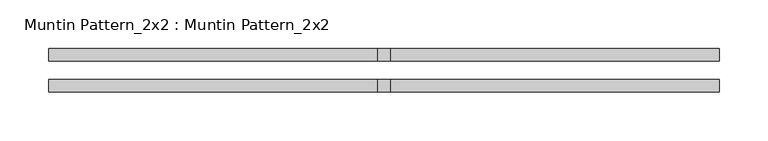
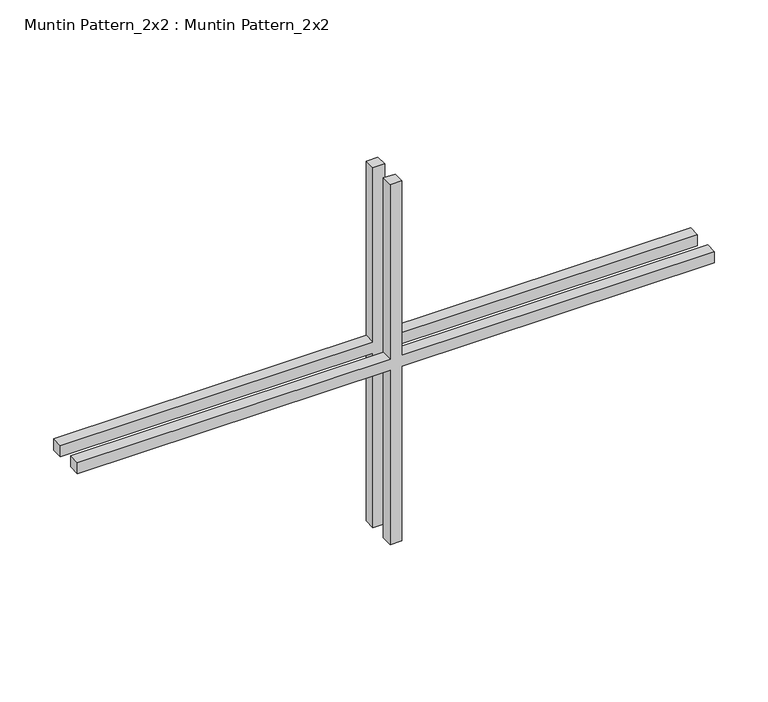
"""IFC4 building model written with IfcOpenShell, lengths in millimetres: proxy geometry, Muntin Pattern_2x2 : Muntin Pattern_2x2."""

import ifcopenshell
import ifcopenshell.guid

model = None  # the IFC model being written
_history = None  # IfcOwnerHistory: only IFC2X3 demands one
_inside = {}  # id of a spatial element -> (the spatial element, [elements in it])
_under = {}  # id of a project, library or spatial element -> (it, [spatial elements below it])
_declared = {}  # id of a project -> (the project, [libraries it declares])
_typed = {}  # id of a type object -> (the type object, [elements of that type])
_made_of = {}  # id of a material, layer set ... -> (it, [elements and type objects made of it])


def new_model(schema):
    """Start an empty IFC model of exactly this schema.

    Asked for "IFC4X3", IfcOpenShell would pick the latest addendum, in which some entities
    have other attributes; the version numbers below select the first issue.
    IFC2X3 requires an IfcOwnerHistory on every rooted entity: one is made here for all.
    """
    global model, _history
    if schema == "IFC4X3":
        model = ifcopenshell.file(schema_version=(4, 3, 0, 0))
    else:
        model = ifcopenshell.file(schema=schema)
    _inside.clear()
    _under.clear()
    _declared.clear()
    _typed.clear()
    _made_of.clear()
    _history = None
    if model.schema == "IFC2X3":
        org = make("IfcOrganization", Name="unknown")
        user = make(
            "IfcPersonAndOrganization",
            ThePerson=make("IfcPerson", FamilyName="unknown"),
            TheOrganization=org,
        )
        app = make(
            "IfcApplication",
            ApplicationDeveloper=org,
            Version="unknown",
            ApplicationFullName="unknown",
            ApplicationIdentifier="unknown",
        )
        _history = make(
            "IfcOwnerHistory",
            OwningUser=user,
            OwningApplication=app,
            ChangeAction="ADDED",
            CreationDate=0,
        )
    return model


def make(cls, **values):
    """One entity of the class cls with the attributes given. An attribute that is None is left unset."""
    return model.create_entity(
        cls, **{name: value for name, value in values.items() if value is not None}
    )


def rooted(cls, **values):
    """An entity with a GlobalId (a new one), such as an element, a storey or a relation."""
    return make(cls, GlobalId=ifcopenshell.guid.new(), OwnerHistory=_history, **values)


def si_unit(unit_type, name, prefix=None):
    """IfcSIUnit, for example si_unit("LENGTHUNIT", "METRE", prefix="MILLI")."""
    return make("IfcSIUnit", UnitType=unit_type, Prefix=prefix, Name=name)


def assignment(units):
    """IfcUnitAssignment: the units of a project."""
    return None if units is None else make("IfcUnitAssignment", Units=units)


def point(xyz):
    """IfcCartesianPoint."""
    return None if xyz is None else make("IfcCartesianPoint", Coordinates=xyz)


def direction(xyz):
    """IfcDirection."""
    return None if xyz is None else make("IfcDirection", DirectionRatios=xyz)


def frame(location, z_axis=None, x_axis=None):
    """IfcAxis2Placement3D, a coordinate frame: its origin and axes. An axis left out is left unset."""
    return make(
        "IfcAxis2Placement3D",
        Location=point(location),
        Axis=direction(z_axis),
        RefDirection=direction(x_axis),
    )


def origin():
    """The frame at (0, 0, 0) with its axes left unset."""
    return frame((0.0, 0.0, 0.0))


def place(relative_to, where):
    """IfcLocalPlacement: puts the frame where relative to a parent placement (None: the world)."""
    return make(
        "IfcLocalPlacement", PlacementRelTo=relative_to, RelativePlacement=where
    )


def context(
    kind, dimensions, precision=None, world=None, true_north=None, identifier=None
):
    """IfcGeometricRepresentationContext, for example the 3D "Model" context."""
    return make(
        "IfcGeometricRepresentationContext",
        ContextIdentifier=identifier,
        ContextType=kind,
        CoordinateSpaceDimension=dimensions,
        Precision=precision,
        WorldCoordinateSystem=world,
        TrueNorth=true_north,
    )


def project(units=None, contexts=None):
    """IfcProject with its units and contexts."""
    return rooted(
        "IfcProject",
        Name="project",
        RepresentationContexts=contexts,
        UnitsInContext=assignment(units),
    )


def spatial(cls, under=None, at=None, **own):
    """A site, building, storey or space (cls), placed at a placement, below another one or the project."""
    s = rooted(cls, ObjectPlacement=at, **own)
    if under is not None:
        _under.setdefault(under.id(), (under, []))[1].append(s)
    return s


def polyline(points):
    """IfcPolyline through the points."""
    return make("IfcPolyline", Points=[point(p) for p in points])


def outline(outer, holes=None, kind="AREA"):
    """IfcArbitraryClosedProfileDef: a profile drawn as a closed curve; with holes, ...WithVoids."""
    if holes is None:
        return make("IfcArbitraryClosedProfileDef", ProfileType=kind, OuterCurve=outer)
    return make(
        "IfcArbitraryProfileDefWithVoids",
        ProfileType=kind,
        OuterCurve=outer,
        InnerCurves=holes,
    )


def extrude(swept, where, along, depth):
    """IfcExtrudedAreaSolid: the profile swept, set in the frame where, extruded along a direction by depth."""
    return make(
        "IfcExtrudedAreaSolid",
        SweptArea=swept,
        Position=where,
        ExtrudedDirection=direction(along),
        Depth=depth,
    )


def shape(context_of_items, identifier, shape_type, items):
    """IfcShapeRepresentation: the items that make up one representation, for example the "Body"."""
    return make(
        "IfcShapeRepresentation",
        ContextOfItems=context_of_items,
        RepresentationIdentifier=identifier,
        RepresentationType=shape_type,
        Items=items,
    )


def source(mapping_origin, context_of_items, identifier, shape_type, items):
    """IfcRepresentationMap: a shape defined once, which mapped items show again and again."""
    return make(
        "IfcRepresentationMap",
        MappingOrigin=mapping_origin,
        MappedRepresentation=shape(context_of_items, identifier, shape_type, items),
    )


def transform(
    local_origin,
    x_axis=None,
    y_axis=None,
    z_axis=None,
    scale=None,
    scale2=None,
    scale3=None,
    uniform=True,
):
    """IfcCartesianTransformationOperator3D, or its non-uniform kind. x_axis, y_axis, z_axis: its Axis1, 2, 3."""
    if uniform:
        return make(
            "IfcCartesianTransformationOperator3D",
            Axis1=direction(x_axis),
            Axis2=direction(y_axis),
            LocalOrigin=point(local_origin),
            Scale=scale,
            Axis3=direction(z_axis),
        )
    return make(
        "IfcCartesianTransformationOperator3DnonUniform",
        Axis1=direction(x_axis),
        Axis2=direction(y_axis),
        LocalOrigin=point(local_origin),
        Scale=scale,
        Axis3=direction(z_axis),
        Scale2=scale2,
        Scale3=scale3,
    )


def mapped(mapping_source, mapping_target):
    """IfcMappedItem: shows the shape of a source again, moved by a transform."""
    return make(
        "IfcMappedItem", MappingSource=mapping_source, MappingTarget=mapping_target
    )


def made_of(thing, what):
    """Note that an element or type object is made of a material, layer set ...; save() writes the relation."""
    if what is not None:
        _made_of.setdefault(what.id(), (what, []))[1].append(thing)
    return thing


def element(
    cls,
    number,
    at=None,
    inside=None,
    cuts=None,
    type_object=None,
    material=None,
    context=None,
    identifier="Body",
    shape_type=None,
    held_by="IfcProductDefinitionShape",
    body=None,
    shapes=None,
    **own,
):
    """One element of the class cls, such as IfcWall. Its Tag is "e" and its number.

    at: its placement. inside: the storey or other place that contains it. cuts: it is an
    opening in that element (IfcRelVoidsElement). A single representation is given by context,
    identifier, shape_type and body (its items); several are given by shapes. held_by: the class
    of the entity that holds the representations. save() writes the other relations.
    """
    e = rooted(cls, Tag="e%d" % number, ObjectPlacement=at, **own)
    if body is not None:
        shapes = [shape(context, identifier, shape_type, body)]
    if shapes is not None:
        e.Representation = make(held_by, Representations=shapes)
    if inside is not None:
        _inside.setdefault(inside.id(), (inside, []))[1].append(e)
    if cuts is not None:
        rooted(
            "IfcRelVoidsElement", RelatingBuildingElement=cuts, RelatedOpeningElement=e
        )
    if type_object is not None:
        _typed.setdefault(type_object.id(), (type_object, []))[1].append(e)
    return made_of(e, material)


def aggregate(whole, parts):
    """IfcRelAggregates: a whole, such as a stair, and the parts it consists of."""
    return rooted("IfcRelAggregates", RelatingObject=whole, RelatedObjects=parts)


def save(model, path):
    """Write the relations noted so far, then the file.

    IfcRelAggregates (storeys below a building ...), IfcRelContainedInSpatialStructure (elements
    in a storey), IfcRelDefinesByType, IfcRelAssociatesMaterial and IfcRelDeclares: one each for
    every whole, place, type object, material and project.
    """
    for whole, parts in _under.values():
        aggregate(whole, parts)
    for where, things in _inside.values():
        rooted(
            "IfcRelContainedInSpatialStructure",
            RelatedElements=things,
            RelatingStructure=where,
        )
    for kind, things in _typed.values():
        rooted("IfcRelDefinesByType", RelatedObjects=things, RelatingType=kind)
    for what, things in _made_of.values():
        rooted("IfcRelAssociatesMaterial", RelatedObjects=things, RelatingMaterial=what)
    for by, libraries in _declared.values():
        rooted("IfcRelDeclares", RelatingContext=by, RelatedDefinitions=libraries)
    model.write(path)


def muntin_pattern_2x2_muntin_pattern_2x2_e664c3e5(model_context):
    return source(origin(), model_context, "Body", "SweptSolid", [
        extrude(outline(polyline([(211.1375, -6.35), (211.1375, -342.9), (198.4375, -342.9), (198.4375, -6.35), (0.0, -6.35), (0.0, 6.35), (198.4375, 6.35), (198.4375, 342.9), (211.1375, 342.9), (211.1375, 6.35), (409.575, 6.35), (409.575, -6.35), (211.1375, -6.35)])), frame((0.0, 9.525, 0.0), z_axis=(0.0, 1.0, 0.0), x_axis=(0.0, 0.0, 1.0)), (0.0, 0.0, 1.0), 12.7),
        extrude(outline(polyline([(211.1375, -6.35), (211.1375, -342.9), (198.4375, -342.9), (198.4375, -6.35), (0.0, -6.35), (0.0, 6.35), (198.4375, 6.35), (198.4375, 342.9), (211.1375, 342.9), (211.1375, 6.35), (409.575, 6.35), (409.575, -6.35), (211.1375, -6.35)])), frame((0.0, -22.225, 0.0), z_axis=(0.0, 1.0, 0.0), x_axis=(0.0, 0.0, 1.0)), (0.0, 0.0, 1.0), 12.7),
    ])


if __name__ == "__main__":
    model = new_model("IFC4")
    model_context = context("Model", 3, world=origin())
    ifc_project = project(units=[si_unit("LENGTHUNIT", "METRE", prefix="MILLI")], contexts=[model_context])
    site = spatial("IfcSite", under=ifc_project)
    building = spatial("IfcBuilding", under=site)
    placement = place(None, origin())
    muntin_pattern_2x2_muntin_pattern_2x2_shape = muntin_pattern_2x2_muntin_pattern_2x2_e664c3e5(model_context)
    element("IfcBuildingElementProxy", 1, Name="Muntin Pattern_2x2 : Muntin Pattern_2x2", ObjectType="Muntin Pattern_2x2 : Muntin Pattern_2x2", at=placement, inside=building, context=model_context, shape_type="MappedRepresentation", body=[
        mapped(muntin_pattern_2x2_muntin_pattern_2x2_shape, transform((0.0, 0.0, 0.0), x_axis=(1.0, 0.0, 0.0), y_axis=(0.0, 1.0, 0.0), z_axis=(0.0, 0.0, 1.0))),
    ])
    save(model, "model.ifc")

# Revit data of these elements
# Type "Muntin Pattern_2x2 : Muntin Pattern_2x2"
#   Width [instance default] = 4' - 0"
#   Thickness = 0' - 0 1/2"
#   Height [instance default] = 4' - 0"
#   Distance = 0' - 0 3/4"
#   Interior Material [instance default] = none
#   Exterior Material [instance default] = none
# Element 1 (IfcBuildingElementProxy, "Muntin Pattern_2x2 : Muntin Pattern_2x2")
#   Width = 2' - 3"
#   Height = 1' - 4 1/8"
#   Interior Material = Wood - Stained
#   Exterior Material = Clad - White
#   Materials on its faces: "Clad - White", "Wood - Stained"
# Materials
#   "Clad - White": class "Wood", colour RGB 242 242 238, transparency 0, Cost = 0
#   "Wood - Stained": class "Wood", colour RGB 224 178 126, transparency 0, Cost = 0
